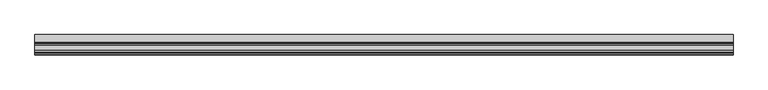
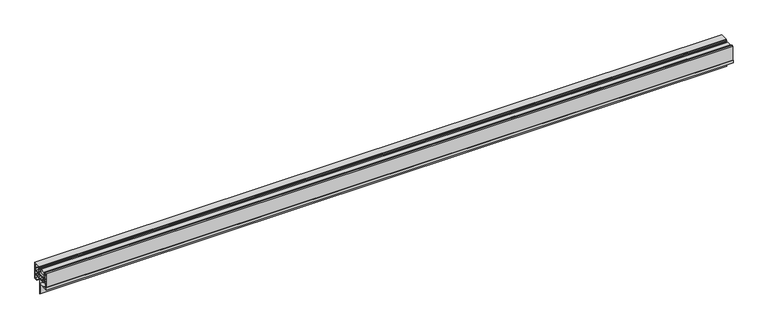
"""IFC4 building model written with IfcOpenShell, lengths in millimetres: proxy geometry, Window frame006 2232 : Window frame006 2232."""

import ifcopenshell
import ifcopenshell.guid

model = None  # the IFC model being written
_history = None  # IfcOwnerHistory: only IFC2X3 demands one
_inside = {}  # id of a spatial element -> (the spatial element, [elements in it])
_under = {}  # id of a project, library or spatial element -> (it, [spatial elements below it])
_declared = {}  # id of a project -> (the project, [libraries it declares])
_typed = {}  # id of a type object -> (the type object, [elements of that type])
_made_of = {}  # id of a material, layer set ... -> (it, [elements and type objects made of it])


def new_model(schema):
    """Start an empty IFC model of exactly this schema.

    Asked for "IFC4X3", IfcOpenShell would pick the latest addendum, in which some entities
    have other attributes; the version numbers below select the first issue.
    IFC2X3 requires an IfcOwnerHistory on every rooted entity: one is made here for all.
    """
    global model, _history
    if schema == "IFC4X3":
        model = ifcopenshell.file(schema_version=(4, 3, 0, 0))
    else:
        model = ifcopenshell.file(schema=schema)
    _inside.clear()
    _under.clear()
    _declared.clear()
    _typed.clear()
    _made_of.clear()
    _history = None
    if model.schema == "IFC2X3":
        org = make("IfcOrganization", Name="unknown")
        user = make(
            "IfcPersonAndOrganization",
            ThePerson=make("IfcPerson", FamilyName="unknown"),
            TheOrganization=org,
        )
        app = make(
            "IfcApplication",
            ApplicationDeveloper=org,
            Version="unknown",
            ApplicationFullName="unknown",
            ApplicationIdentifier="unknown",
        )
        _history = make(
            "IfcOwnerHistory",
            OwningUser=user,
            OwningApplication=app,
            ChangeAction="ADDED",
            CreationDate=0,
        )
    return model


def make(cls, **values):
    """One entity of the class cls with the attributes given. An attribute that is None is left unset."""
    return model.create_entity(
        cls, **{name: value for name, value in values.items() if value is not None}
    )


def rooted(cls, **values):
    """An entity with a GlobalId (a new one), such as an element, a storey or a relation."""
    return make(cls, GlobalId=ifcopenshell.guid.new(), OwnerHistory=_history, **values)


def si_unit(unit_type, name, prefix=None):
    """IfcSIUnit, for example si_unit("LENGTHUNIT", "METRE", prefix="MILLI")."""
    return make("IfcSIUnit", UnitType=unit_type, Prefix=prefix, Name=name)


def assignment(units):
    """IfcUnitAssignment: the units of a project."""
    return None if units is None else make("IfcUnitAssignment", Units=units)


def point(xyz):
    """IfcCartesianPoint."""
    return None if xyz is None else make("IfcCartesianPoint", Coordinates=xyz)


def direction(xyz):
    """IfcDirection."""
    return None if xyz is None else make("IfcDirection", DirectionRatios=xyz)


def frame(location, z_axis=None, x_axis=None):
    """IfcAxis2Placement3D, a coordinate frame: its origin and axes. An axis left out is left unset."""
    return make(
        "IfcAxis2Placement3D",
        Location=point(location),
        Axis=direction(z_axis),
        RefDirection=direction(x_axis),
    )


def origin():
    """The frame at (0, 0, 0) with its axes left unset."""
    return frame((0.0, 0.0, 0.0))


def place(relative_to, where):
    """IfcLocalPlacement: puts the frame where relative to a parent placement (None: the world)."""
    return make(
        "IfcLocalPlacement", PlacementRelTo=relative_to, RelativePlacement=where
    )


def context(
    kind, dimensions, precision=None, world=None, true_north=None, identifier=None
):
    """IfcGeometricRepresentationContext, for example the 3D "Model" context."""
    return make(
        "IfcGeometricRepresentationContext",
        ContextIdentifier=identifier,
        ContextType=kind,
        CoordinateSpaceDimension=dimensions,
        Precision=precision,
        WorldCoordinateSystem=world,
        TrueNorth=true_north,
    )


def project(units=None, contexts=None):
    """IfcProject with its units and contexts."""
    return rooted(
        "IfcProject",
        Name="project",
        RepresentationContexts=contexts,
        UnitsInContext=assignment(units),
    )


def spatial(cls, under=None, at=None, **own):
    """A site, building, storey or space (cls), placed at a placement, below another one or the project."""
    s = rooted(cls, ObjectPlacement=at, **own)
    if under is not None:
        _under.setdefault(under.id(), (under, []))[1].append(s)
    return s


def polyline(points):
    """IfcPolyline through the points."""
    return make("IfcPolyline", Points=[point(p) for p in points])


def outline(outer, holes=None, kind="AREA"):
    """IfcArbitraryClosedProfileDef: a profile drawn as a closed curve; with holes, ...WithVoids."""
    if holes is None:
        return make("IfcArbitraryClosedProfileDef", ProfileType=kind, OuterCurve=outer)
    return make(
        "IfcArbitraryProfileDefWithVoids",
        ProfileType=kind,
        OuterCurve=outer,
        InnerCurves=holes,
    )


def extrude(swept, where, along, depth):
    """IfcExtrudedAreaSolid: the profile swept, set in the frame where, extruded along a direction by depth."""
    return make(
        "IfcExtrudedAreaSolid",
        SweptArea=swept,
        Position=where,
        ExtrudedDirection=direction(along),
        Depth=depth,
    )


def shape(context_of_items, identifier, shape_type, items):
    """IfcShapeRepresentation: the items that make up one representation, for example the "Body"."""
    return make(
        "IfcShapeRepresentation",
        ContextOfItems=context_of_items,
        RepresentationIdentifier=identifier,
        RepresentationType=shape_type,
        Items=items,
    )


def source(mapping_origin, context_of_items, identifier, shape_type, items):
    """IfcRepresentationMap: a shape defined once, which mapped items show again and again."""
    return make(
        "IfcRepresentationMap",
        MappingOrigin=mapping_origin,
        MappedRepresentation=shape(context_of_items, identifier, shape_type, items),
    )


def transform(
    local_origin,
    x_axis=None,
    y_axis=None,
    z_axis=None,
    scale=None,
    scale2=None,
    scale3=None,
    uniform=True,
):
    """IfcCartesianTransformationOperator3D, or its non-uniform kind. x_axis, y_axis, z_axis: its Axis1, 2, 3."""
    if uniform:
        return make(
            "IfcCartesianTransformationOperator3D",
            Axis1=direction(x_axis),
            Axis2=direction(y_axis),
            LocalOrigin=point(local_origin),
            Scale=scale,
            Axis3=direction(z_axis),
        )
    return make(
        "IfcCartesianTransformationOperator3DnonUniform",
        Axis1=direction(x_axis),
        Axis2=direction(y_axis),
        LocalOrigin=point(local_origin),
        Scale=scale,
        Axis3=direction(z_axis),
        Scale2=scale2,
        Scale3=scale3,
    )


def mapped(mapping_source, mapping_target):
    """IfcMappedItem: shows the shape of a source again, moved by a transform."""
    return make(
        "IfcMappedItem", MappingSource=mapping_source, MappingTarget=mapping_target
    )


def made_of(thing, what):
    """Note that an element or type object is made of a material, layer set ...; save() writes the relation."""
    if what is not None:
        _made_of.setdefault(what.id(), (what, []))[1].append(thing)
    return thing


def element(
    cls,
    number,
    at=None,
    inside=None,
    cuts=None,
    type_object=None,
    material=None,
    context=None,
    identifier="Body",
    shape_type=None,
    held_by="IfcProductDefinitionShape",
    body=None,
    shapes=None,
    **own,
):
    """One element of the class cls, such as IfcWall. Its Tag is "e" and its number.

    at: its placement. inside: the storey or other place that contains it. cuts: it is an
    opening in that element (IfcRelVoidsElement). A single representation is given by context,
    identifier, shape_type and body (its items); several are given by shapes. held_by: the class
    of the entity that holds the representations. save() writes the other relations.
    """
    e = rooted(cls, Tag="e%d" % number, ObjectPlacement=at, **own)
    if body is not None:
        shapes = [shape(context, identifier, shape_type, body)]
    if shapes is not None:
        e.Representation = make(held_by, Representations=shapes)
    if inside is not None:
        _inside.setdefault(inside.id(), (inside, []))[1].append(e)
    if cuts is not None:
        rooted(
            "IfcRelVoidsElement", RelatingBuildingElement=cuts, RelatedOpeningElement=e
        )
    if type_object is not None:
        _typed.setdefault(type_object.id(), (type_object, []))[1].append(e)
    return made_of(e, material)


def aggregate(whole, parts):
    """IfcRelAggregates: a whole, such as a stair, and the parts it consists of."""
    return rooted("IfcRelAggregates", RelatingObject=whole, RelatedObjects=parts)


def save(model, path):
    """Write the relations noted so far, then the file.

    IfcRelAggregates (storeys below a building ...), IfcRelContainedInSpatialStructure (elements
    in a storey), IfcRelDefinesByType, IfcRelAssociatesMaterial and IfcRelDeclares: one each for
    every whole, place, type object, material and project.
    """
    for whole, parts in _under.values():
        aggregate(whole, parts)
    for where, things in _inside.values():
        rooted(
            "IfcRelContainedInSpatialStructure",
            RelatedElements=things,
            RelatingStructure=where,
        )
    for kind, things in _typed.values():
        rooted("IfcRelDefinesByType", RelatedObjects=things, RelatingType=kind)
    for what, things in _made_of.values():
        rooted("IfcRelAssociatesMaterial", RelatedObjects=things, RelatingMaterial=what)
    for by, libraries in _declared.values():
        rooted("IfcRelDeclares", RelatingContext=by, RelatedDefinitions=libraries)
    model.write(path)


def generic_models_94aafbfd(model_context):
    return source(origin(), model_context, "Body", "SweptSolid", [
        extrude(outline(polyline([(10410.6588026, 40821.2566334), (10410.6588026, 40823.6696334), (10412.8850166, 40823.6696334), (10413.3087579, 40826.1285263), (10414.6621229, 40826.1285263), (10415.2977621, 40823.2665501), (10415.2977621, 40821.4051872), (10414.635235, 40818.8149696), (10413.4611227, 40818.8149696), (10412.8857105, 40821.2566334), (10410.6588026, 40821.2566334)])), frame((3694.2883192, 0.0, 0.0), z_axis=(1.0, 0.0, 0.0), x_axis=(0.0, 1.0, 0.0)), (0.0, 0.0, 1.0), 2000.0),
        extrude(outline(polyline([(10445.4060026, 40823.6868625), (10445.4060026, 40821.2738625), (10443.1797886, 40821.2738625), (10442.7560473, 40818.8149696), (10441.4026824, 40818.8149696), (10440.7670432, 40821.6769458), (10440.7670432, 40823.5383087), (10441.4295703, 40826.1285263), (10442.6036826, 40826.1285263), (10443.1790948, 40823.6868625), (10445.4060026, 40823.6868625)])), frame((3694.2883192, 0.0, 0.0), z_axis=(1.0, 0.0, 0.0), x_axis=(0.0, 1.0, 0.0)), (0.0, 0.0, 1.0), 2000.0),
        extrude(outline(polyline([(3694.2883192, 10421.6443026), (3694.2883192, 10434.4205026), (5694.2883192, 10434.4205026), (5694.2883192, 10421.6443026), (3694.2883192, 10421.6443026)])), frame((0.0, 0.0, 40813.5903625), z_axis=(0.0, 0.0, 1.0), x_axis=(1.0, 0.0, 0.0)), (0.0, 0.0, 1.0), 9.525),
        extrude(outline(polyline([(10426.7016425, 40805.8433625), (10426.7016425, 40807.7119447), (10419.7882638, 40807.7119447), (10419.7882638, 40804.0145625), (10412.9702026, 40804.0145625), (10412.9702026, 40807.2931991), (10414.872119, 40807.2931991), (10414.872119, 40812.064471), (10416.637419, 40813.5903625), (10440.7451026, 40813.5903625), (10440.7451026, 40805.8433625), (10426.7016425, 40805.8433625)])), frame((3694.2883192, 0.0, 0.0), z_axis=(1.0, 0.0, 0.0), x_axis=(0.0, 1.0, 0.0)), (0.0, 0.0, 1.0), 2000.0),
        extrude(outline(polyline([(10462.3610631, 40808.8405625), (10463.2880173, 40806.7829834), (10462.2265149, 40805.1664558), (10460.9383822, 40805.1664558), (10460.9383822, 40810.2375625), (10464.3290026, 40810.2375625), (10464.3290026, 40824.8933625), (10447.0570026, 40824.8933625), (10447.0570026, 40804.4463625), (10423.0393446, 40804.4463625), (10423.0393446, 40805.8179625), (10445.6600026, 40805.8179625), (10445.6600026, 40818.6703625), (10443.1200026, 40818.6703625), (10443.1200026, 40820.8466583), (10444.3883807, 40820.8466583), (10444.3883807, 40819.9403625), (10445.6600026, 40819.9403625), (10445.6600026, 40825.0203625), (10444.3883807, 40825.0203625), (10444.3883807, 40824.0988632), (10443.1200026, 40824.0988632), (10443.1200026, 40826.2903625), (10465.7260026, 40826.2903625), (10465.7260026, 40808.8405625), (10462.3610631, 40808.8405625)])), frame((3694.2883192, 0.0, 0.0), z_axis=(1.0, 0.0, 0.0), x_axis=(0.0, 1.0, 0.0)), (0.0, 0.0, 1.0), 2000.0),
        extrude(outline(polyline([(10424.5780026, 40792.4321625), (10424.5780026, 40801.9825625), (10419.9887905, 40801.9825625), (10419.9887905, 40804.0145625), (10421.5291892, 40804.0145625), (10421.5291892, 40807.1895625), (10425.9768772, 40807.1895625), (10425.9768772, 40805.8433625), (10423.0393446, 40805.8433625), (10423.0393446, 40804.0145625), (10463.6940026, 40804.0145625), (10463.6940026, 40806.2748048), (10462.438716, 40808.8405625), (10465.7260026, 40808.8405625), (10465.7260026, 40777.2175625), (10455.2358026, 40777.2175625), (10455.2358026, 40779.2495625), (10463.6940026, 40779.2495625), (10463.4400026, 40790.4001625), (10441.9008026, 40790.4001625), (10441.9008026, 40746.8700298), (10440.3260031, 40746.8700298), (10440.3260031, 40790.4001625), (10420.7680026, 40790.4001625), (10420.7680026, 40793.9693733), (10422.0343473, 40793.9693733), (10422.0343473, 40792.4321625), (10424.5780026, 40792.4321625)]), holes=[polyline([(10459.7037468, 40792.4321625), (10463.1860026, 40792.4321625), (10463.1860026, 40801.9825625), (10459.7037468, 40801.9825625), (10459.7037468, 40800.8395625), (10449.7649031, 40800.8395625), (10449.7649031, 40801.9825625), (10446.1345473, 40801.9825625), (10446.1345473, 40800.8395625), (10440.9864026, 40800.8395625), (10440.9864026, 40801.9825625), (10434.1726294, 40801.9825625), (10434.1726294, 40800.8395625), (10426.6100026, 40800.8395625), (10426.6100026, 40793.5751625), (10430.5720244, 40793.5751625), (10430.5720244, 40792.4321625), (10439.5580617, 40792.4321625), (10439.5580617, 40793.5751625), (10446.1345473, 40793.5751625), (10446.1345473, 40792.4321625), (10454.3772498, 40792.4321625), (10454.3772498, 40793.5751625), (10459.7037468, 40793.5751625), (10459.7037468, 40792.4321625)])]), frame((3694.2883192, 0.0, 0.0), z_axis=(1.0, 0.0, 0.0), x_axis=(0.0, 1.0, 0.0)), (0.0, 0.0, 1.0), 2000.0),
        extrude(outline(polyline([(10408.5760026, 40777.2175625), (10440.3260026, 40777.2175625), (10440.3260026, 40745.4675625), (10439.3100026, 40745.4675625), (10439.3100026, 40776.2015625), (10407.5600026, 40776.2015625), (10407.5600026, 40783.5675625), (10408.5760026, 40783.5675625), (10408.5760026, 40777.2175625)])), frame((3694.2883192, 0.0, 0.0), z_axis=(1.0, 0.0, 0.0), x_axis=(0.0, 1.0, 0.0)), (0.0, 0.0, 1.0), 2000.0),
        extrude(outline(polyline([(10408.5760026, 40826.2903625), (10412.9702026, 40826.2903625), (10412.9702026, 40824.1609092), (10411.7002026, 40824.1609092), (10411.7002026, 40825.0203625), (10410.4302026, 40825.0203625), (10410.4302026, 40819.9403625), (10411.7002026, 40819.9403625), (10411.7002026, 40820.7984291), (10412.9702026, 40820.7984291), (10412.9702026, 40804.0145625), (10415.1972148, 40804.0145625), (10415.1972148, 40801.9825625), (10410.6080026, 40801.9825625), (10410.6080026, 40792.4321625), (10413.073783, 40792.4321625), (10413.073783, 40793.9693733), (10414.4180026, 40793.9693733), (10414.4180026, 40790.4001625), (10410.6080026, 40790.4001625), (10410.6080026, 40779.2495625), (10418.8122026, 40779.2495625), (10418.8122026, 40777.2175625), (10408.5760026, 40777.2175625), (10408.5760026, 40826.2903625)])), frame((3694.2883192, 0.0, 0.0), z_axis=(1.0, 0.0, 0.0), x_axis=(0.0, 1.0, 0.0)), (0.0, 0.0, 1.0), 2000.0),
    ])


if __name__ == "__main__":
    model = new_model("IFC4")
    model_context = context("Model", 3, world=origin())
    ifc_project = project(units=[si_unit("LENGTHUNIT", "METRE", prefix="MILLI")], contexts=[model_context])
    site = spatial("IfcSite", under=ifc_project)
    building = spatial("IfcBuilding", under=site)
    placement = place(None, origin())
    generic_models_shape = generic_models_94aafbfd(model_context)
    element("IfcBuildingElementProxy", 1, Name="Window frame006 2232 : Window frame006 2232", ObjectType="Window frame006 2232 : Window frame006 2232", at=placement, inside=building, context=model_context, shape_type="MappedRepresentation", body=[
        mapped(generic_models_shape, transform((0.0, 0.0, 0.0), x_axis=(1.0, 0.0, 0.0), y_axis=(0.0, 1.0, 0.0), z_axis=(0.0, 0.0, 1.0))),
    ])
    save(model, "model.ifc")

# Revit data of these elements
# Type "Window frame006 2232 : Window frame006 2232"
#   NameOverride = "Window frame006"
# Element 1 (IfcBuildingElementProxy, "Window frame006 2232 : Window frame006 2232")
#   Materials on its faces: "FLEETWOOD SERIES 250-T-04 FIXED UNIT WINDOW FRAME"
# Materials
#   "FLEETWOOD SERIES 250-T-04 FIXED UNIT WINDOW FRAME": class "Unassigned", colour RGB 128 128 128, transparency 0
